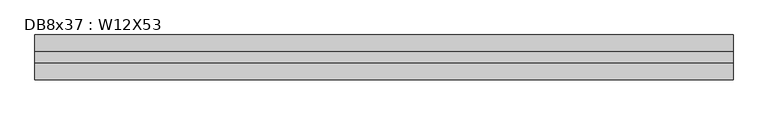
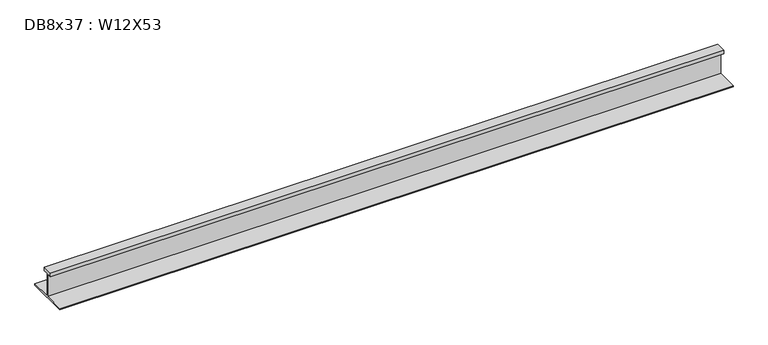
"""IFC4 building model written with IfcOpenShell, lengths in millimetres: beam geometry, DB8x37 : W12X53."""

from ifc_helpers import new_model, si_unit, frame, origin, place, context, project, spatial, polyline, outline, extrude, source, transform, mapped, element, save


def db8x37_w12x53_a48d096f(model_context):
    return source(origin(), model_context, "Body", "SweptSolid", [
        extrude(outline(polyline([(38.1, 145.415), (38.1, 120.015), (2.921, 120.015), (2.921, -48.4505), (152.4, -48.4505), (152.4, -58.1025), (-152.4, -58.1025), (-152.4, -48.4505), (-2.921, -48.4505), (-2.921, 120.015), (-38.1, 120.015), (-38.1, 145.415), (38.1, 145.415)])), frame((-2391.029, 0.0, 0.0), z_axis=(1.0, 0.0, 0.0), x_axis=(0.0, 1.0, 0.0)), (0.0, 0.0, 1.0), 4754.499),
    ])


if __name__ == "__main__":
    model = new_model("IFC4")
    model_context = context("Model", 3, world=origin())
    ifc_project = project(units=[si_unit("LENGTHUNIT", "METRE", prefix="MILLI")], contexts=[model_context])
    site = spatial("IfcSite", under=ifc_project)
    building = spatial("IfcBuilding", under=site)
    placement = place(None, origin())
    db8x37_w12x53_shape = db8x37_w12x53_a48d096f(model_context)
    element("IfcBeam", 1, ObjectType="DB8x37 : W12X53", at=placement, inside=building, context=model_context, shape_type="MappedRepresentation", body=[
        mapped(db8x37_w12x53_shape, transform((0.0, 0.0, 0.0), x_axis=(1.0, 0.0, 0.0), y_axis=(0.0, 1.0, 0.0), z_axis=(0.0, 0.0, 1.0))),
    ])
    save(model, "model.ifc")

# Revit data of these elements
# Type "DB8x37 : W12X53"
#   Assembly Code = "B10"
#   W = 53
#   Length [instance default] = 5' - 0"
#   bf = 0' - 10"
#   d = 1' - 0.1"
#   k = 0' - 1 3/8"
#   k2 = 0' - 0.8"
#   tf = 0' - 0.575"
#   tw = 0' - 0.345"
#   A = 0.108333 SF
#   Structural Material [instance default] = Steel ASTM A992
# Element 1 (IfcBeam, "DB8x37 : W12X53")
#   Materials on its faces: "Steel ASTM A992"
# Materials
#   "Steel ASTM A992": class "Metal", colour RGB 199 199 199, transparency 0, Description = "Structural steel 50ksi", Cost = 0
